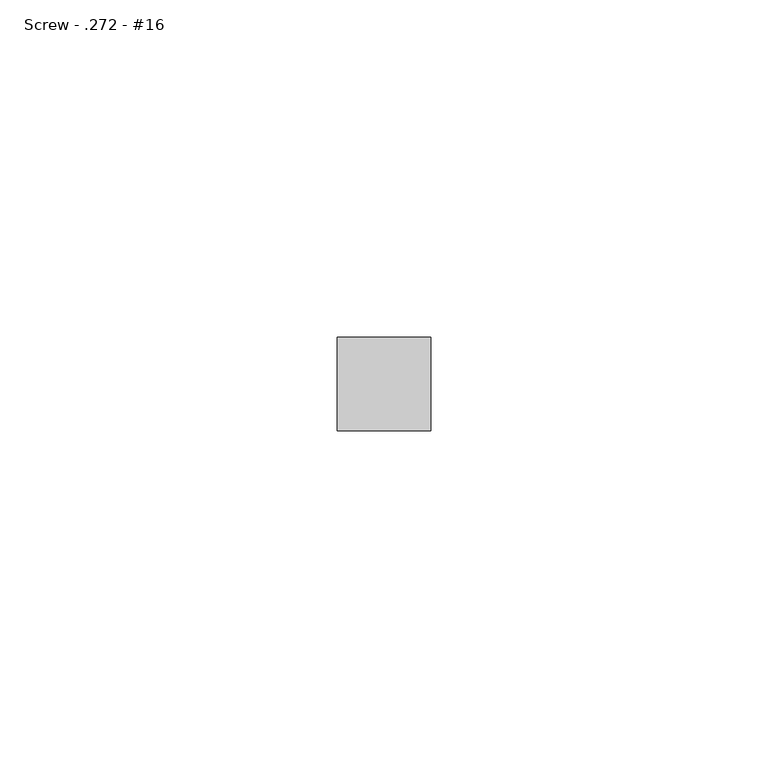
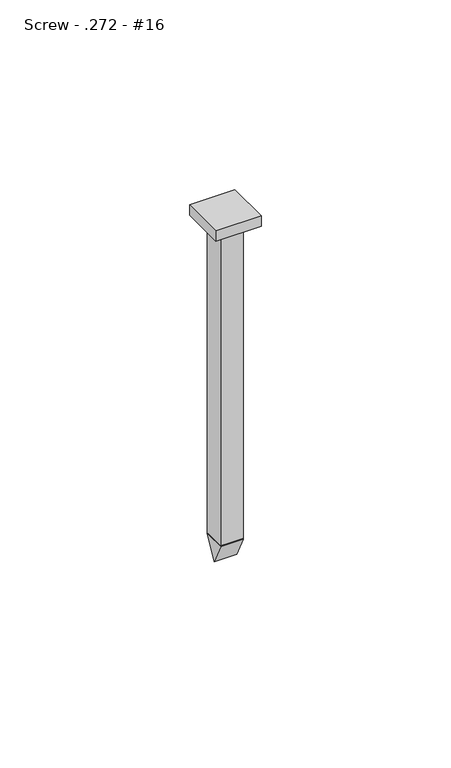
"""IFC4 building model written with IfcOpenShell, lengths in millimetres: fastener geometry, 060523 - W_P_C - Fastenings - Generic - SQUARE : Screw - .272 - #16."""

from ifc_helpers import new_model, si_unit, frame, origin, origin_with_axes, place, context, project, spatial, polyline, outline, extrude, source, transform, mapped, element, save


def screw_272_16_5d55c0d5(model_context):
    return source(origin(), model_context, "Body", "SweptSolid", [
        extrude(outline(polyline([(0.0, -108.5088), (-3.4544, -101.6), (3.4544, -101.6), (0.0, -108.5088)])), frame((-3.4544, 0.0, 0.0), z_axis=(1.0, 0.0, 0.0), x_axis=(0.0, 1.0, 0.0)), (0.0, 0.0, 1.0), 6.9088),
        extrude(outline(polyline([(-6.9088, -6.9088), (-6.9088, 6.9088), (6.9088, 6.9088), (6.9088, -6.9088), (-6.9088, -6.9088)])), origin_with_axes(), (0.0, 0.0, 1.0), 3.4544),
        extrude(outline(polyline([(-3.4544, 3.4544), (3.4544, 3.4544), (3.4544, -3.4544), (-3.4544, -3.4544), (-3.4544, 3.4544)])), frame((0.0, 0.0, -101.6), z_axis=(0.0, 0.0, 1.0), x_axis=(1.0, 0.0, 0.0)), (0.0, 0.0, 1.0), 101.6),
    ])


if __name__ == "__main__":
    model = new_model("IFC4")
    model_context = context("Model", 3, world=origin())
    ifc_project = project(units=[si_unit("LENGTHUNIT", "METRE", prefix="MILLI")], contexts=[model_context])
    site = spatial("IfcSite", under=ifc_project)
    building = spatial("IfcBuilding", under=site)
    placement = place(None, origin())
    screw_272_16_shape = screw_272_16_5d55c0d5(model_context)
    element("IfcFastener", 1, ObjectType="060523 - W_P_C - Fastenings - Generic - SQUARE : Screw - .272 - #16", at=placement, inside=building, context=model_context, shape_type="MappedRepresentation", body=[
        mapped(screw_272_16_shape, transform((0.0, 0.0, 0.0), x_axis=(1.0, 0.0, 0.0), y_axis=(0.0, 1.0, 0.0), z_axis=(0.0, 0.0, 1.0))),
    ])
    save(model, "model.ifc")

# Revit data of these elements
# Type "060523 - W_P_C - Fastenings - Generic - SQUARE : Screw - .272 - #16"
#   Washer_Thickness = 0' - 0.00333"
#   Washer Radius = 0' - 0.146"
#   Washer Offset - Head = 0' - 0"
#   Washer Offset = 0' - 0"
#   Thickness_of_Substrate [instance default] = 0' - 1"
#   Side = 0' - 0 37/64"
#   Radius = 0' - 0.136"
#   Length [instance default] = 0' - 4"
#   Head Size = 0' - 1"
#   Head Radius = 0' - 0 1/2"
#   Head Height = 0' - 0.01"
#   Double Diameter = 0' - 0.544"
#   Diameter = 0' - 0.272"
#   Default Elevation = 4' - 0"
#   Washer_Nut_Visibility = no
#   Washer_Head_Visibility = no
#   Round_Head_Visibility = yes
#   Point Visibility = yes
#   Nut_Visibility = no
#   Hex_Head_Visiblilty = no
#   Washer Material = none
#   Bolt Material (Size) = AT SILL - FASTENER AT 24" O.C.
# Materials
#   "AT SILL - FASTENER AT 24\" O.C.": class "Generic", colour RGB 120 120 120, transparency 0, Cost = 0
